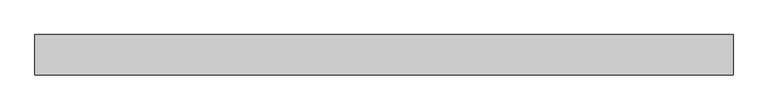
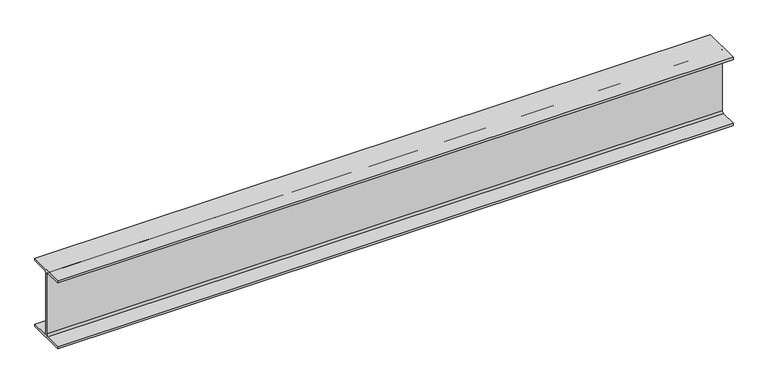
"""IFC4 building model written with IfcOpenShell, lengths in millimetres: beam geometry, Old_Steel Beam_H-KSD3502 : H_SB_ASB_H-200×200x8x12."""

import ifcopenshell
import ifcopenshell.guid

model = None  # the IFC model being written
_history = None  # IfcOwnerHistory: only IFC2X3 demands one
_inside = {}  # id of a spatial element -> (the spatial element, [elements in it])
_under = {}  # id of a project, library or spatial element -> (it, [spatial elements below it])
_declared = {}  # id of a project -> (the project, [libraries it declares])
_typed = {}  # id of a type object -> (the type object, [elements of that type])
_made_of = {}  # id of a material, layer set ... -> (it, [elements and type objects made of it])


def new_model(schema):
    """Start an empty IFC model of exactly this schema.

    Asked for "IFC4X3", IfcOpenShell would pick the latest addendum, in which some entities
    have other attributes; the version numbers below select the first issue.
    IFC2X3 requires an IfcOwnerHistory on every rooted entity: one is made here for all.
    """
    global model, _history
    if schema == "IFC4X3":
        model = ifcopenshell.file(schema_version=(4, 3, 0, 0))
    else:
        model = ifcopenshell.file(schema=schema)
    _inside.clear()
    _under.clear()
    _declared.clear()
    _typed.clear()
    _made_of.clear()
    _history = None
    if model.schema == "IFC2X3":
        org = make("IfcOrganization", Name="unknown")
        user = make(
            "IfcPersonAndOrganization",
            ThePerson=make("IfcPerson", FamilyName="unknown"),
            TheOrganization=org,
        )
        app = make(
            "IfcApplication",
            ApplicationDeveloper=org,
            Version="unknown",
            ApplicationFullName="unknown",
            ApplicationIdentifier="unknown",
        )
        _history = make(
            "IfcOwnerHistory",
            OwningUser=user,
            OwningApplication=app,
            ChangeAction="ADDED",
            CreationDate=0,
        )
    return model


def make(cls, **values):
    """One entity of the class cls with the attributes given. An attribute that is None is left unset."""
    return model.create_entity(
        cls, **{name: value for name, value in values.items() if value is not None}
    )


def rooted(cls, **values):
    """An entity with a GlobalId (a new one), such as an element, a storey or a relation."""
    return make(cls, GlobalId=ifcopenshell.guid.new(), OwnerHistory=_history, **values)


def si_unit(unit_type, name, prefix=None):
    """IfcSIUnit, for example si_unit("LENGTHUNIT", "METRE", prefix="MILLI")."""
    return make("IfcSIUnit", UnitType=unit_type, Prefix=prefix, Name=name)


def assignment(units):
    """IfcUnitAssignment: the units of a project."""
    return None if units is None else make("IfcUnitAssignment", Units=units)


def point(xyz):
    """IfcCartesianPoint."""
    return None if xyz is None else make("IfcCartesianPoint", Coordinates=xyz)


def direction(xyz):
    """IfcDirection."""
    return None if xyz is None else make("IfcDirection", DirectionRatios=xyz)


def frame(location, z_axis=None, x_axis=None):
    """IfcAxis2Placement3D, a coordinate frame: its origin and axes. An axis left out is left unset."""
    return make(
        "IfcAxis2Placement3D",
        Location=point(location),
        Axis=direction(z_axis),
        RefDirection=direction(x_axis),
    )


def frame_2d(location, x_axis=None):
    """IfcAxis2Placement2D, a coordinate frame in the plane: its origin and x axis."""
    return make(
        "IfcAxis2Placement2D", Location=point(location), RefDirection=direction(x_axis)
    )


def origin():
    """The frame at (0, 0, 0) with its axes left unset."""
    return frame((0.0, 0.0, 0.0))


def place(relative_to, where):
    """IfcLocalPlacement: puts the frame where relative to a parent placement (None: the world)."""
    return make(
        "IfcLocalPlacement", PlacementRelTo=relative_to, RelativePlacement=where
    )


def context(
    kind, dimensions, precision=None, world=None, true_north=None, identifier=None
):
    """IfcGeometricRepresentationContext, for example the 3D "Model" context."""
    return make(
        "IfcGeometricRepresentationContext",
        ContextIdentifier=identifier,
        ContextType=kind,
        CoordinateSpaceDimension=dimensions,
        Precision=precision,
        WorldCoordinateSystem=world,
        TrueNorth=true_north,
    )


def project(units=None, contexts=None):
    """IfcProject with its units and contexts."""
    return rooted(
        "IfcProject",
        Name="project",
        RepresentationContexts=contexts,
        UnitsInContext=assignment(units),
    )


def spatial(cls, under=None, at=None, **own):
    """A site, building, storey or space (cls), placed at a placement, below another one or the project."""
    s = rooted(cls, ObjectPlacement=at, **own)
    if under is not None:
        _under.setdefault(under.id(), (under, []))[1].append(s)
    return s


def polyline(points):
    """IfcPolyline through the points."""
    return make("IfcPolyline", Points=[point(p) for p in points])


def circle_curve(where, radius):
    """IfcCircle in the frame where."""
    return make("IfcCircle", Position=where, Radius=radius)


def trimmed(basis, trim1, trim2, sense, master):
    """IfcTrimmedCurve: the piece of a basis curve between two trims."""
    return make(
        "IfcTrimmedCurve",
        BasisCurve=basis,
        Trim1=trim1,
        Trim2=trim2,
        SenseAgreement=sense,
        MasterRepresentation=master,
    )


def segment(curve, same_sense, transition):
    """IfcCompositeCurveSegment."""
    return make(
        "IfcCompositeCurveSegment",
        Transition=transition,
        SameSense=same_sense,
        ParentCurve=curve,
    )


def composite_curve(segments, self_intersect=None):
    """IfcCompositeCurve: segments joined end to end."""
    return make("IfcCompositeCurve", Segments=segments, SelfIntersect=self_intersect)


def outline(outer, holes=None, kind="AREA"):
    """IfcArbitraryClosedProfileDef: a profile drawn as a closed curve; with holes, ...WithVoids."""
    if holes is None:
        return make("IfcArbitraryClosedProfileDef", ProfileType=kind, OuterCurve=outer)
    return make(
        "IfcArbitraryProfileDefWithVoids",
        ProfileType=kind,
        OuterCurve=outer,
        InnerCurves=holes,
    )


def extrude(swept, where, along, depth):
    """IfcExtrudedAreaSolid: the profile swept, set in the frame where, extruded along a direction by depth."""
    return make(
        "IfcExtrudedAreaSolid",
        SweptArea=swept,
        Position=where,
        ExtrudedDirection=direction(along),
        Depth=depth,
    )


def shape(context_of_items, identifier, shape_type, items):
    """IfcShapeRepresentation: the items that make up one representation, for example the "Body"."""
    return make(
        "IfcShapeRepresentation",
        ContextOfItems=context_of_items,
        RepresentationIdentifier=identifier,
        RepresentationType=shape_type,
        Items=items,
    )


def source(mapping_origin, context_of_items, identifier, shape_type, items):
    """IfcRepresentationMap: a shape defined once, which mapped items show again and again."""
    return make(
        "IfcRepresentationMap",
        MappingOrigin=mapping_origin,
        MappedRepresentation=shape(context_of_items, identifier, shape_type, items),
    )


def transform(
    local_origin,
    x_axis=None,
    y_axis=None,
    z_axis=None,
    scale=None,
    scale2=None,
    scale3=None,
    uniform=True,
):
    """IfcCartesianTransformationOperator3D, or its non-uniform kind. x_axis, y_axis, z_axis: its Axis1, 2, 3."""
    if uniform:
        return make(
            "IfcCartesianTransformationOperator3D",
            Axis1=direction(x_axis),
            Axis2=direction(y_axis),
            LocalOrigin=point(local_origin),
            Scale=scale,
            Axis3=direction(z_axis),
        )
    return make(
        "IfcCartesianTransformationOperator3DnonUniform",
        Axis1=direction(x_axis),
        Axis2=direction(y_axis),
        LocalOrigin=point(local_origin),
        Scale=scale,
        Axis3=direction(z_axis),
        Scale2=scale2,
        Scale3=scale3,
    )


def mapped(mapping_source, mapping_target):
    """IfcMappedItem: shows the shape of a source again, moved by a transform."""
    return make(
        "IfcMappedItem", MappingSource=mapping_source, MappingTarget=mapping_target
    )


def made_of(thing, what):
    """Note that an element or type object is made of a material, layer set ...; save() writes the relation."""
    if what is not None:
        _made_of.setdefault(what.id(), (what, []))[1].append(thing)
    return thing


def element(
    cls,
    number,
    at=None,
    inside=None,
    cuts=None,
    type_object=None,
    material=None,
    context=None,
    identifier="Body",
    shape_type=None,
    held_by="IfcProductDefinitionShape",
    body=None,
    shapes=None,
    **own,
):
    """One element of the class cls, such as IfcWall. Its Tag is "e" and its number.

    at: its placement. inside: the storey or other place that contains it. cuts: it is an
    opening in that element (IfcRelVoidsElement). A single representation is given by context,
    identifier, shape_type and body (its items); several are given by shapes. held_by: the class
    of the entity that holds the representations. save() writes the other relations.
    """
    e = rooted(cls, Tag="e%d" % number, ObjectPlacement=at, **own)
    if body is not None:
        shapes = [shape(context, identifier, shape_type, body)]
    if shapes is not None:
        e.Representation = make(held_by, Representations=shapes)
    if inside is not None:
        _inside.setdefault(inside.id(), (inside, []))[1].append(e)
    if cuts is not None:
        rooted(
            "IfcRelVoidsElement", RelatingBuildingElement=cuts, RelatedOpeningElement=e
        )
    if type_object is not None:
        _typed.setdefault(type_object.id(), (type_object, []))[1].append(e)
    return made_of(e, material)


def aggregate(whole, parts):
    """IfcRelAggregates: a whole, such as a stair, and the parts it consists of."""
    return rooted("IfcRelAggregates", RelatingObject=whole, RelatedObjects=parts)


def save(model, path):
    """Write the relations noted so far, then the file.

    IfcRelAggregates (storeys below a building ...), IfcRelContainedInSpatialStructure (elements
    in a storey), IfcRelDefinesByType, IfcRelAssociatesMaterial and IfcRelDeclares: one each for
    every whole, place, type object, material and project.
    """
    for whole, parts in _under.values():
        aggregate(whole, parts)
    for where, things in _inside.values():
        rooted(
            "IfcRelContainedInSpatialStructure",
            RelatedElements=things,
            RelatingStructure=where,
        )
    for kind, things in _typed.values():
        rooted("IfcRelDefinesByType", RelatedObjects=things, RelatingType=kind)
    for what, things in _made_of.values():
        rooted("IfcRelAssociatesMaterial", RelatedObjects=things, RelatingMaterial=what)
    for by, libraries in _declared.values():
        rooted("IfcRelDeclares", RelatingContext=by, RelatedDefinitions=libraries)
    model.write(path)


def beam_c1fe6c0d(model_context):
    return source(origin(), model_context, "Body", "SweptSolid", [
        extrude(outline(composite_curve([segment(polyline([(82.5, -141.5), (82.5, -151.7), (-82.5, -151.7), (-82.5, -141.5), (-11.9, -141.5)]), True, "CONTINUOUS"), segment(trimmed(circle_curve(frame_2d((-11.9, -132.6)), 8.9), [point((-11.9, -141.5))], [point((-3.0, -132.6))], True, "CARTESIAN"), True, "CONTINUOUS"), segment(polyline([(-3.0, -132.6), (-3.0, 132.6)]), True, "CONTINUOUS"), segment(trimmed(circle_curve(frame_2d((-11.9, 132.6)), 8.9), [point((-3.0, 132.6))], [point((-11.9, 141.5))], True, "CARTESIAN"), True, "CONTINUOUS"), segment(polyline([(-11.9, 141.5), (-82.5, 141.5), (-82.5, 151.7), (82.5, 151.7), (82.5, 141.5), (11.9, 141.5)]), True, "CONTINUOUS"), segment(trimmed(circle_curve(frame_2d((11.9, 132.6)), 8.9), [point((11.9, 141.5))], [point((3.0, 132.6))], True, "CARTESIAN"), True, "CONTINUOUS"), segment(polyline([(3.0, 132.6), (3.0, -132.6)]), True, "CONTINUOUS"), segment(trimmed(circle_curve(frame_2d((11.9, -132.6)), 8.9), [point((3.0, -132.6))], [point((11.9, -141.5))], True, "CARTESIAN"), True, "CONTINUOUS"), segment(polyline([(11.9, -141.5), (82.5, -141.5)]), True, "CONTINUOUS")], self_intersect=False)), frame((-1432.8225766, 0.0, 0.0), z_axis=(1.0, 0.0, 0.0), x_axis=(0.0, 1.0, 0.0)), (0.0, 0.0, 1.0), 2841.3927387),
    ])


if __name__ == "__main__":
    model = new_model("IFC4")
    model_context = context("Model", 3, world=origin())
    ifc_project = project(units=[si_unit("LENGTHUNIT", "METRE", prefix="MILLI")], contexts=[model_context])
    site = spatial("IfcSite", under=ifc_project)
    building = spatial("IfcBuilding", under=site)
    placement = place(None, origin())
    beam_shape = beam_c1fe6c0d(model_context)
    element("IfcBeam", 1, ObjectType="Old_Steel Beam_H-KSD3502 : H_SB_ASB_H-200×200x8x12", at=placement, inside=building, context=model_context, shape_type="MappedRepresentation", body=[
        mapped(beam_shape, transform((0.0, 0.0, 0.0), x_axis=(1.0, 0.0, 0.0), y_axis=(0.0, 1.0, 0.0), z_axis=(0.0, 0.0, 1.0))),
    ])
    save(model, "model.ifc")

# Revit data of these elements
# Type "Old_Steel Beam_H-KSD3502 : H_SB_ASB_H-200×200x8x12"
#   Width = 20.0 cm
#   Web Thickness = 0.8 cm
#   Web Fillet = 1.3 cm
#   Warping Constant = 141376.0 cm⁶
#   Torsional Moment of Inertia = 26.2485 cm⁴
#   Torsional Modulus = 1.0 cm³
#   Section Area = 63.53 cm²
#   Plastic Modulus weak axis = 244.0 cm³
#   Plastic Modulus strong axis = 525.0 cm³
#   Perimeter = 1.16 m²/m
#   Nominal Weight = 49.90 kgf/m
#   Moment of Inertia weak axis = 1600.00 cm⁴
#   Moment of Inertia strong axis = 4720.00 cm⁴
#   Height = 20.0 cm
#   Flange Thickness = 1.2 cm
#   Elastic Modulus weak axis = 160.0 cm³
#   Elastic Modulus strong axis = 472.0 cm³
#   Centroid Vertical = 10.0 cm
#   Centroid Horizontal = 10.0 cm
#   Length [instance default] = 1.5240 m
#   Structural Material [instance default] = Steel, 45-345
#   Assembly Code = ""
# Element 1 (IfcBeam, "Old_Steel Beam_H-KSD3502 : H_SB_ASB_H-200×200x8x12")
#   Structural Material = none
# Materials
#   "Steel, 45-345": class "Metal", colour RGB 189 187 185, transparency 0, Description = "Steel 345 MPa", Cost = 0
